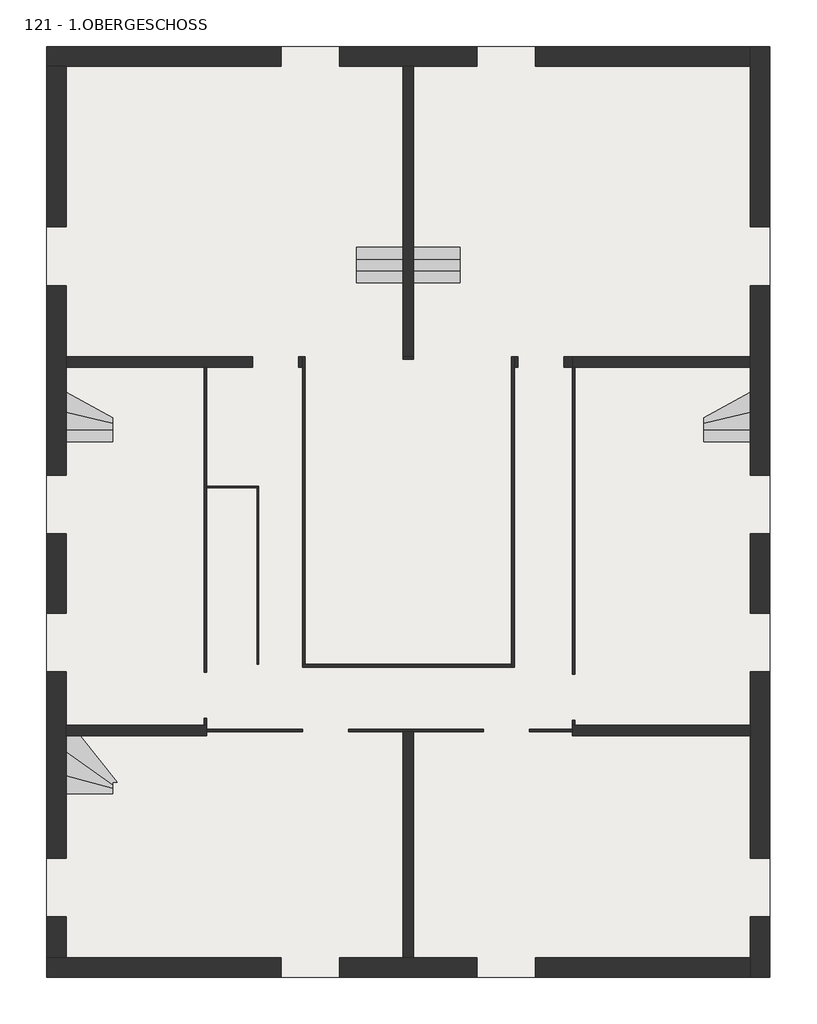
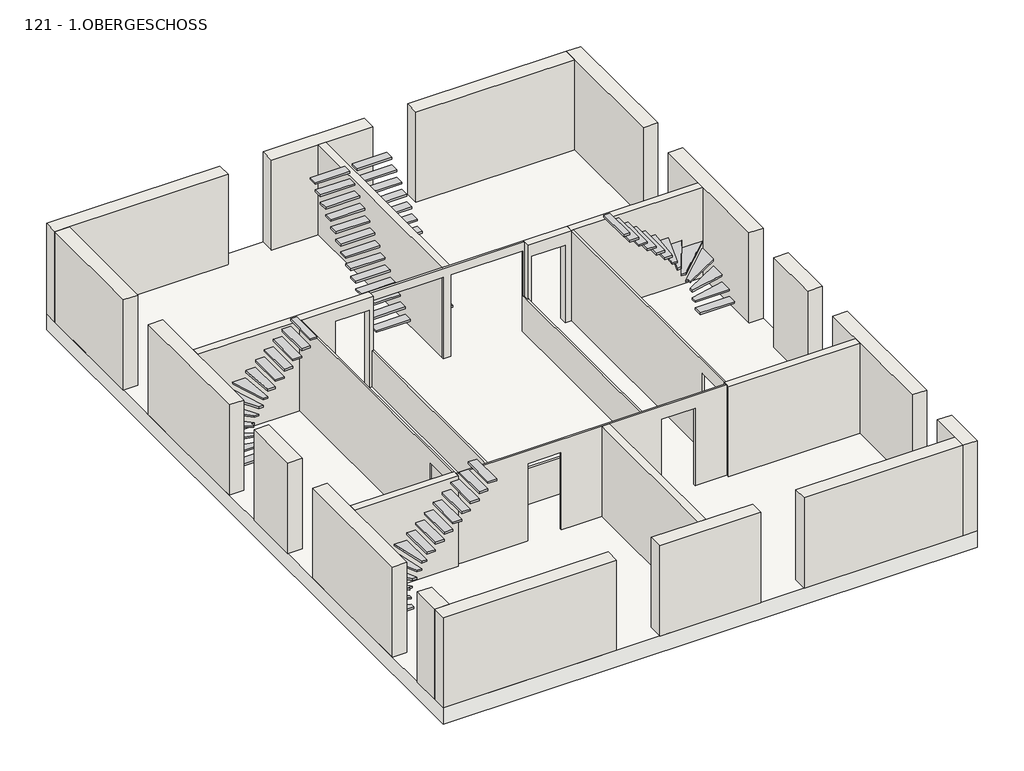
# One storey: 20 walls, 10 stairs, 1 slab.
# Revit data of these elements (continued)
# Type "  97010 :   97010" (continued)
#   Allright_Bauteil_ID = "0121Tre0785086959"
#   Material = "Stahlbeton"
#   Objektname = "Treppe"
#   NameOverride = " "
#   ThermalTransmittance = 0.0000 BTU/(h·ft²·°F)
#   NosingLength = 0.000 m
#   NumberOfRiser = 14
#   NumberOfTreads = 14
#   RiserHeight = 2.000 m
#   TreadLength = 2.300 m
#   IsExternal = no
#   FireExit = no
#   HandicapAccessible = no
#   HasNonSkidSurface = no
# Type "  97882 :   97882"
#   Abrechnungsart = "St"
#   Allright_Bauteil_ID = "0121Tre0785065280"
#   Codetext = "TR-MASSIV-GER\\"
#   Material = "Stahlbeton"
#   Objektname = "Treppe"
#   NameOverride = " "
#   Reference = "STB-Treppe"
#   ThermalTransmittance = 0.0000 BTU/(h·ft²·°F)
#   NosingLength = 0.000 m
#   NumberOfRiser = 14
#   NumberOfTreads = 13
#   RiserHeight = 2.021 m
#   TreadLength = 2.300 m
#   IsExternal = no
#   FireExit = no
#   HandicapAccessible = no
#   HasNonSkidSurface = no
# Type "  98300 :   98300"
#   Abrechnungsart = "St"
#   Allright_Bauteil_ID = "0121Tre0785065278"
#   Codetext = "TR-MASSIV-GER\\"
#   Material = "Stahlbeton"
#   Objektname = "Treppe"
#   NameOverride = " "
#   Reference = "STB-Treppe"
#   ThermalTransmittance = 0.0000 BTU/(h·ft²·°F)
#   NosingLength = 0.000 m
#   NumberOfRiser = 14
#   NumberOfTreads = 13
#   RiserHeight = 2.021 m
#   TreadLength = 2.300 m
#   IsExternal = no
#   FireExit = no
#   HandicapAccessible = no
#   HasNonSkidSurface = no
# Type "  98728 :   98728"
#   Abrechnungsart = "St"
#   Allright_Bauteil_ID = "0121Tre0785070507"
#   Material = "Stahlbeton"
#   Objektname = "Treppe"
#   NameOverride = " "
#   ThermalTransmittance = 0.0000 BTU/(h·ft²·°F)
#   NosingLength = 0.000 m
#   NumberOfRiser = 14
#   NumberOfTreads = 13
#   RiserHeight = 2.021 m
#   TreadLength = 2.300 m
#   IsExternal = no
#   FireExit = no
#   HandicapAccessible = no
#   HasNonSkidSurface = no
# Type "  99154 :   99154"
#   Abrechnungsart = "St"
#   Allright_Bauteil_ID = "0121Tre0785070829"
#   Material = "Stahlbeton"
#   Objektname = "Treppe"
#   NameOverride = " "
#   ThermalTransmittance = 0.0000 BTU/(h·ft²·°F)
#   NosingLength = 0.000 m
#   NumberOfRiser = 14
#   NumberOfTreads = 13
#   RiserHeight = 2.021 m
#   TreadLength = 2.300 m
#   IsExternal = no
#   FireExit = no
#   HandicapAccessible = no
#   HasNonSkidSurface = no
# Type "  149542 :   149542"
#   Abrechnungsart = "St"
#   Allright_Bauteil_ID = "0131Tre0659044515"
#   Material = "Stahlbeton"
#   Objektname = "Treppe"
#   NameOverride = " "
#   ThermalTransmittance = 0.0000 BTU/(h·ft²·°F)
#   NosingLength = 0.000 m
#   NumberOfRiser = 14
#   NumberOfTreads = 14
#   RiserHeight = 2.000 m
#   TreadLength = 2.300 m
#   IsExternal = no
#   FireExit = no
#   HandicapAccessible = no
#   HasNonSkidSurface = no
# Type "  150414 :   150414"
#   Abrechnungsart = "St"
#   Allright_Bauteil_ID = "0131Tre0659044575"
#   Codetext = "TR-MASSIV-GER\\"
#   Material = "Stahlbeton"
#   Objektname = "Treppe"
#   NameOverride = " "
#   Reference = "STB-Treppe"
#   ThermalTransmittance = 0.0000 BTU/(h·ft²·°F)
#   NosingLength = 0.000 m
#   NumberOfRiser = 14
#   NumberOfTreads = 13
#   RiserHeight = 2.021 m
#   TreadLength = 2.300 m
#   IsExternal = no
#   FireExit = no
#   HandicapAccessible = no
#   HasNonSkidSurface = no
# Type "  150832 :   150832"
#   Abrechnungsart = "St"
#   Allright_Bauteil_ID = "0131Tre0659044593"
#   Codetext = "TR-MASSIV-GER\\"
#   Material = "Stahlbeton"
#   Objektname = "Treppe"
#   NameOverride = " "
#   Reference = "STB-Treppe"
#   ThermalTransmittance = 0.0000 BTU/(h·ft²·°F)
#   NosingLength = 0.000 m
#   NumberOfRiser = 14
#   NumberOfTreads = 13
#   RiserHeight = 2.021 m
#   TreadLength = 2.300 m
#   IsExternal = no
#   FireExit = no
#   HandicapAccessible = no
#   HasNonSkidSurface = no
# Type "  151260 :   151260"
#   Abrechnungsart = "St"
#   Allright_Bauteil_ID = "0131Tre0659044533"
#   Material = "Stahlbeton"
#   Objektname = "Treppe"
#   NameOverride = " "
#   ThermalTransmittance = 0.0000 BTU/(h·ft²·°F)
#   NosingLength = 0.000 m
#   NumberOfRiser = 14
#   NumberOfTreads = 13
#   RiserHeight = 2.021 m
#   TreadLength = 2.300 m
#   IsExternal = no
#   FireExit = no
#   HandicapAccessible = no
#   HasNonSkidSurface = no
# Type "  151686 :   151686"
#   Abrechnungsart = "St"
#   Allright_Bauteil_ID = "0131Tre0659044570"
#   Material = "Stahlbeton"
#   Objektname = "Treppe"
#   NameOverride = " "
#   ThermalTransmittance = 0.0000 BTU/(h·ft²·°F)
#   NosingLength = 0.000 m
#   NumberOfRiser = 14
#   NumberOfTreads = 13
#   RiserHeight = 2.021 m
#   TreadLength = 2.300 m
#   IsExternal = no
#   FireExit = no
#   HandicapAccessible = no
#   HasNonSkidSurface = no
# Type " :1166"
#   Layers, outside or top first: 0.050 m "glas" (function 1)
# Type "Holzwand:1150"
#   ThermalTransmittance = 0.0000 BTU/(h·ft²·°F)
#   Combustible = no
#   Compartmentation = no
#   Layers, outside or top first: 0.200 m "holzschalung" (function 1)
# Type "Holzwand:1151"
#   ThermalTransmittance = 0.0000 BTU/(h·ft²·°F)
#   Combustible = no
#   Compartmentation = no
#   Layers, outside or top first: 0.200 m "holzschalung" (function 1)
# Type "Holzwand:1153"
#   ThermalTransmittance = 0.0000 BTU/(h·ft²·°F)
#   Combustible = no
#   Compartmentation = no
#   Layers, outside or top first: 0.200 m "holzschalung" (function 1)
# Type "Holzwand:1154"
#   ThermalTransmittance = 0.0000 BTU/(h·ft²·°F)
#   Combustible = no
#   Compartmentation = no
#   Layers, outside or top first: 0.030 m "holzschalung" (function 1)
# Type "Holzwand:1155"
#   ThermalTransmittance = 0.0000 BTU/(h·ft²·°F)
#   Combustible = no
#   Compartmentation = no
#   Layers, outside or top first: 0.030 m "holzschalung" (function 1)
# Type "1186 Atriumwand"
#   Layers, outside or top first: 0.050 m "holzschalung" (function 1)
# Type "Holzwand:1157"
#   ThermalTransmittance = 0.0000 BTU/(h·ft²·°F)
#   Combustible = no
#   Compartmentation = no
#   Layers, outside or top first: 0.200 m "holzschalung" (function 1)
# Type "Holzwand:1160"
#   ThermalTransmittance = 0.0000 BTU/(h·ft²·°F)
#   Combustible = no
#   Compartmentation = no
#   Layers, outside or top first: 0.200 m "holzschalung" (function 1)
# Type "Holzwand:1162"
#   ThermalTransmittance = 0.0000 BTU/(h·ft²·°F)
#   Combustible = no
#   Compartmentation = no
#   Layers, outside or top first: 0.200 m "holzschalung" (function 1)
# Type "Holzwand:1163"
#   ThermalTransmittance = 0.0000 BTU/(h·ft²·°F)
#   Combustible = no
#   Compartmentation = no
#   Layers, outside or top first: 0.200 m "holzschalung" (function 1)
# Type " :1167"
#   Layers, outside or top first: 0.050 m "holzschalung" (function 1)
# Type " :1168"
#   Layers, outside or top first: 0.050 m "holzschalung" (function 1)
# Type " :1169"
#   Layers, outside or top first: 0.050 m "holzschalung" (function 1)
# Type "1141 Aussenwand"
#   Layers, outside or top first: 0.380 m "holzschalung" (function 1)
# Element 1 (IfcSlab, "Holzdecke 176 : Holzdecke 176")
#   IFC Predefined Type = "FLOOR"
#   Export to IFC As = "ifcslab"
#   IfcGUID = "1_9Us2eVX4OuIZjhNyqdxW"
#   Phase Created = New Construction
#   Materials on its faces: "holzschalung"
# Element 2 (IfcStair, "  97010 :   97010")
#   IFC Predefined Type = "NOTDEFINED"
#   Export to IFC As = "ifcstair"
#   IfcGUID = "2ccaodaeb6QgHPV1d4NBnA"
#   Phase Created = New Construction
#   Materials on its faces: "weiss"
# Element 3 (IfcStair, "  97882 :   97882")
#   IFC Predefined Type = "STRAIGHT_RUN_STAIR"
#   Export to IFC As = "ifcstair"
#   IfcGUID = "1nghyUHoH9yBc_lxkBTUjw"
#   Phase Created = New Construction
#   Materials on its faces: "weiss"
# Element 4 (IfcStair, "  98300 :   98300")
#   IFC Predefined Type = "STRAIGHT_RUN_STAIR"
#   Export to IFC As = "ifcstair"
#   IfcGUID = "2AC_Gmfhz1LvYwUyPOxWan"
#   Phase Created = New Construction
#   Materials on its faces: "weiss"
# Element 5 (IfcStair, "  98728 :   98728")
#   IFC Predefined Type = "NOTDEFINED"
#   Export to IFC As = "ifcstair"
#   IfcGUID = "04Edcgbk9CPwWYiYhycXFf"
#   Phase Created = New Construction
#   Materials on its faces: "weiss"
# Element 6 (IfcStair, "  99154 :   99154")
#   IFC Predefined Type = "NOTDEFINED"
#   Export to IFC As = "ifcstair"
#   IfcGUID = "1azVXxNdn2POY9VYN93ccY"
#   Phase Created = New Construction
#   Materials on its faces: "weiss"
# Element 7 (IfcStair, "  149542 :   149542")
#   IFC Predefined Type = "NOTDEFINED"
#   Export to IFC As = "ifcstair"
#   IfcGUID = "1sH4rJKnLAFOtHPnXrLkif"
#   Phase Created = New Construction
#   Materials on its faces: "weiss"
# Element 8 (IfcStair, "  150414 :   150414")
#   IFC Predefined Type = "STRAIGHT_RUN_STAIR"
#   Export to IFC As = "ifcstair"
#   IfcGUID = "3fdccs_Mj1YAyFFpBc3gyk"
#   Phase Created = New Construction
#   Materials on its faces: "weiss"
# Element 9 (IfcStair, "  150832 :   150832")
#   IFC Predefined Type = "STRAIGHT_RUN_STAIR"
#   Export to IFC As = "ifcstair"
#   IfcGUID = "2szmEZdbD3KBDvfX1Sa6Vh"
#   Phase Created = New Construction
#   Materials on its faces: "weiss"
# Element 10 (IfcStair, "  151260 :   151260")
#   IFC Predefined Type = "NOTDEFINED"
#   Export to IFC As = "ifcstair"
#   IfcGUID = "1YKyaFTbr8YR41yGjubBsl"
#   Phase Created = New Construction
#   Materials on its faces: "weiss"
# Element 11 (IfcStair, "  151686 :   151686")
#   IFC Predefined Type = "NOTDEFINED"
#   Export to IFC As = "ifcstair"
#   IfcGUID = "2KPGRYHzzCygzBebAeLtPz"
#   Phase Created = New Construction
#   Materials on its faces: "weiss"
# Element 12 (IfcWall, " :1166")
#   Export to IFC As = "ifcwall"
#   IfcGUID = "0t2qqx1kvDZPNPdKl4bfzP"
#   NameOverride = " "
#   Abrechnungsart = "m³"
#   Allright_Bauteil_ID = "0121HWa0785064296"
#   Layer #1:Object Layer Attributes #1:Abrechnungsart = "m²"
#   Layer #1:Object Layer Attributes #1:Allright_Bauteil_ID = "0121Wa 0785064386"
#   Layer #1:Object Layer Attributes #1:Gewerk = "Zimmer- und Holzbauarbeiten"
#   Layer #1:Object Layer Attributes #1:Material = "k.Ausw."
#   Layer #1:Object Layer Attributes #1:Objektname = "Wand"
#   Layer #1:Object Layer Attributes #1:Status = "Neubau"
#   MEP Wandtyp = "HO-WA-HSW\\"
#   Objektname = "Gesamtwand"
#   built-in parameter 1001111 = 0.505 m
#   Top Offset = 0.000 m
#   Base Offset = 0.505 m
#   Unconnected Height = 2.500 m
#   wall height = 2.500 m
#   Layer #1:Object Layer Attributes #1:2D Interaktion = yes
#   Phase Created = New Construction
#   Base Constraint = 121 - 1.OBERGESCHOSS
#   Materials on its faces: "glas"
# Element 13 (IfcWall, "Holzwand:1150")
#   Export to IFC As = "ifcwall"
#   IfcGUID = "3nZ5Mon9nBjwoRgvyoor9a"
#   NameOverride = "Holzwand"
#   Abrechnungsart = "St"
#   Allright_Bauteil_ID = "0121HWa0785065367"
#   Bezeichnung = "Holzwand"
#   Layer #1:Object Layer Attributes #1:Abrechnungsart = "m²"
#   Layer #1:Object Layer Attributes #1:Allright_Bauteil_ID = "0121Wa 0785065369"
#   Layer #1:Object Layer Attributes #1:Bezeichnung = "Holzwand"
#   Layer #1:Object Layer Attributes #1:Codetext = "HO-WI-HSW\\"
#   Layer #1:Object Layer Attributes #1:Gewerk = "Zimmer- und Holzbauarbeiten"
#   Layer #1:Object Layer Attributes #1:Material = "Holz"
#   Layer #1:Object Layer Attributes #1:Objektname = "Wand"
#   Layer #1:Object Layer Attributes #1:Reference = "Holzwand"
#   Layer #1:Object Layer Attributes #1:Status = "Neubau"
#   MEP Wandtyp = "HO-WA-HSW\\"
#   Objektname = "Gesamtwand"
#   Reference = "Holzwand"
#   Status = "NEW"
#   built-in parameter 1001111 = 0.505 m
#   Top Offset = 0.000 m
#   Base Offset = 0.505 m
#   Unconnected Height = 2.500 m
#   wall height = 2.500 m
#   Layer #1:Object Layer Attributes #1:U-Wert = 0
#   Layer #1:Object Layer Attributes #1:2D Interaktion = yes
#   Layer #1:Object Layer Attributes #1:Außenbauteil = no
#   Layer #1:Object Layer Attributes #1:Brandabschnittsdefinierendes Bauteil = no
#   Layer #1:Object Layer Attributes #1:Brennbares Material = no
#   Layer #1:Object Layer Attributes #1:Raumhohe Wand = yes
#   Layer #1:Object Layer Attributes #1:Tragendes Bauteil = yes
#   ExtendToStructure = yes
#   IsExternal = no
#   LoadBearing = yes
#   Phase Created = New Construction
#   Base Constraint = 121 - 1.OBERGESCHOSS
#   Materials on its faces: "holzschalung"
# Element 14 (IfcWall, "Holzwand:1151")
#   Export to IFC As = "ifcwall"
#   IfcGUID = "3jE1E$NFj7vAP$vn70kdrt"
#   NameOverride = "Holzwand"
#   Abrechnungsart = "St"
#   Allright_Bauteil_ID = "0121HWa0785066899"
#   Bezeichnung = "Holzwand"
#   Layer #1:Object Layer Attributes #1:Abrechnungsart = "m²"
#   Layer #1:Object Layer Attributes #1:Allright_Bauteil_ID = "0121Wa 0785066901"
#   Layer #1:Object Layer Attributes #1:Bezeichnung = "Holzwand"
#   Layer #1:Object Layer Attributes #1:Codetext = "HO-WI-HSW\\"
#   Layer #1:Object Layer Attributes #1:Gewerk = "Zimmer- und Holzbauarbeiten"
#   Layer #1:Object Layer Attributes #1:Material = "Holz"
#   Layer #1:Object Layer Attributes #1:Objektname = "Wand"
#   Layer #1:Object Layer Attributes #1:Reference = "Holzwand"
#   Layer #1:Object Layer Attributes #1:Status = "Neubau"
#   MEP Wandtyp = "HO-WA-HSW\\"
#   Objektname = "Gesamtwand"
#   Reference = "Holzwand"
#   Status = "NEW"
#   built-in parameter 1001111 = 0.505 m
#   Top Offset = 0.000 m
#   Base Offset = 0.505 m
#   Unconnected Height = 2.500 m
#   wall height = 2.500 m
#   Layer #1:Object Layer Attributes #1:U-Wert = 0
#   Layer #1:Object Layer Attributes #1:2D Interaktion = yes
#   Layer #1:Object Layer Attributes #1:Außenbauteil = no
#   Layer #1:Object Layer Attributes #1:Brandabschnittsdefinierendes Bauteil = no
#   Layer #1:Object Layer Attributes #1:Brennbares Material = no
#   Layer #1:Object Layer Attributes #1:Raumhohe Wand = yes
#   Layer #1:Object Layer Attributes #1:Tragendes Bauteil = yes
#   ExtendToStructure = yes
#   IsExternal = no
#   LoadBearing = yes
#   Phase Created = New Construction
#   Base Constraint = 121 - 1.OBERGESCHOSS
#   Materials on its faces: "holzschalung"
# Element 15 (IfcWall, "Holzwand:1153")
#   Export to IFC As = "ifcwall"
#   IfcGUID = "1Zhxv5EALB9e6_$pCtUEXg"
#   NameOverride = "Holzwand"
#   Abrechnungsart = "St"
#   Allright_Bauteil_ID = "0121HWa0785065540"
#   Bezeichnung = "Holzwand"
#   Layer #1:Object Layer Attributes #1:Abrechnungsart = "m²"
#   Layer #1:Object Layer Attributes #1:Allright_Bauteil_ID = "0121Wa 0785065541"
#   Layer #1:Object Layer Attributes #1:Bezeichnung = "Holzwand"
#   Layer #1:Object Layer Attributes #1:Codetext = "HO-WI-HSW\\"
#   Layer #1:Object Layer Attributes #1:Gewerk = "Zimmer- und Holzbauarbeiten"
#   Layer #1:Object Layer Attributes #1:Material = "Holz"
#   Layer #1:Object Layer Attributes #1:Objektname = "Wand"
#   Layer #1:Object Layer Attributes #1:Reference = "Holzwand"
#   Layer #1:Object Layer Attributes #1:Status = "Neubau"
#   MEP Wandtyp = "HO-WA-HSW\\"
#   Objektname = "Gesamtwand"
#   Reference = "Holzwand"
#   Status = "NEW"
#   built-in parameter 1001111 = 0.505 m
#   Top Offset = 0.000 m
#   Base Offset = 0.505 m
#   Unconnected Height = 2.500 m
#   wall height = 2.500 m
#   Layer #1:Object Layer Attributes #1:U-Wert = 0
#   Layer #1:Object Layer Attributes #1:2D Interaktion = yes
#   Layer #1:Object Layer Attributes #1:Außenbauteil = no
#   Layer #1:Object Layer Attributes #1:Brandabschnittsdefinierendes Bauteil = no
#   Layer #1:Object Layer Attributes #1:Brennbares Material = no
#   Layer #1:Object Layer Attributes #1:Raumhohe Wand = yes
#   Layer #1:Object Layer Attributes #1:Tragendes Bauteil = yes
#   ExtendToStructure = yes
#   IsExternal = no
#   LoadBearing = yes
#   Phase Created = New Construction
#   Base Constraint = 121 - 1.OBERGESCHOSS
#   Materials on its faces: "holzschalung"
# Element 16 (IfcWall, "Holzwand:1154")
#   Export to IFC As = "ifcwall"
#   IfcGUID = "2MsVq3EJn0K8wHdQ6uoxnd"
#   NameOverride = "Holzwand"
#   Abrechnungsart = "St"
#   Allright_Bauteil_ID = "0121HWa0785067355"
#   Bezeichnung = "Holzwand"
#   Layer #1:Object Layer Attributes #1:Abrechnungsart = "m²"
#   Layer #1:Object Layer Attributes #1:Allright_Bauteil_ID = "0121Wa 0785067356"
#   Layer #1:Object Layer Attributes #1:Codetext = "HO-WI-HSW\\"
#   Layer #1:Object Layer Attributes #1:Gewerk = "Zimmer- und Holzbauarbeiten"
#   Layer #1:Object Layer Attributes #1:Material = "Holz"
#   Layer #1:Object Layer Attributes #1:Objektname = "Wand"
#   Layer #1:Object Layer Attributes #1:Reference = "Holzwand"
#   Layer #1:Object Layer Attributes #1:Status = "Neubau"
#   MEP Wandtyp = "HO-WA-HSW\\"
#   Objektname = "Gesamtwand"
#   Reference = "Holzwand"
#   Status = "NEW"
#   built-in parameter 1001111 = 0.505 m
#   Top Offset = 0.000 m
#   Base Offset = 0.505 m
#   Unconnected Height = 1.000 m
#   wall height = 1.000 m
#   Layer #1:Object Layer Attributes #1:U-Wert = 0
#   Layer #1:Object Layer Attributes #1:2D Interaktion = yes
#   Layer #1:Object Layer Attributes #1:Außenbauteil = no
#   Layer #1:Object Layer Attributes #1:Brandabschnittsdefinierendes Bauteil = no
#   Layer #1:Object Layer Attributes #1:Brennbares Material = no
#   Layer #1:Object Layer Attributes #1:Raumhohe Wand = yes
#   ExtendToStructure = yes
#   IsExternal = no
#   LoadBearing = yes
#   Phase Created = New Construction
#   Base Constraint = 121 - 1.OBERGESCHOSS
#   Materials on its faces: "holzschalung"
# Element 17 (IfcWall, "Holzwand:1155")
#   Export to IFC As = "ifcwall"
#   IfcGUID = "1F_ySrDsP9oP3MqXymSTVO"
#   NameOverride = "Holzwand"
#   Abrechnungsart = "St"
#   Allright_Bauteil_ID = "0121HWa0785067347"
#   Bezeichnung = "Holzwand"
#   Layer #1:Object Layer Attributes #1:Abrechnungsart = "m²"
#   Layer #1:Object Layer Attributes #1:Allright_Bauteil_ID = "0121Wa 0785067348"
#   Layer #1:Object Layer Attributes #1:Codetext = "HO-WI-HSW\\"
#   Layer #1:Object Layer Attributes #1:Gewerk = "Zimmer- und Holzbauarbeiten"
#   Layer #1:Object Layer Attributes #1:Material = "Holz"
#   Layer #1:Object Layer Attributes #1:Objektname = "Wand"
#   Layer #1:Object Layer Attributes #1:Reference = "Holzwand"
#   Layer #1:Object Layer Attributes #1:Status = "Neubau"
#   MEP Wandtyp = "HO-WA-HSW\\"
#   Objektname = "Gesamtwand"
#   Reference = "Holzwand"
#   Status = "NEW"
#   built-in parameter 1001111 = 0.505 m
#   Top Offset = 0.000 m
#   Base Offset = 0.505 m
#   Unconnected Height = 1.000 m
#   wall height = 1.000 m
#   Layer #1:Object Layer Attributes #1:U-Wert = 0
#   Layer #1:Object Layer Attributes #1:2D Interaktion = yes
#   Layer #1:Object Layer Attributes #1:Außenbauteil = no
#   Layer #1:Object Layer Attributes #1:Brandabschnittsdefinierendes Bauteil = no
#   Layer #1:Object Layer Attributes #1:Brennbares Material = no
#   Layer #1:Object Layer Attributes #1:Raumhohe Wand = yes
#   ExtendToStructure = yes
#   IsExternal = no
#   LoadBearing = yes
#   Phase Created = New Construction
#   Base Constraint = 121 - 1.OBERGESCHOSS
#   Materials on its faces: "holzschalung"
# Element 18 (IfcWall, "1186 Atriumwand")
#   Export to IFC As = "ifcwall"
#   IfcGUID = "0gtwZwppj1pObqyI7HY41_"
#   NameOverride = "Holzwand"
#   Abrechnungsart = "St"
#   Allright_Bauteil_ID = "0121HWa0785064323"
#   Bezeichnung = "Holzwand"
#   Layer #1:Object Layer Attributes #1:Abrechnungsart = "m²"
#   Layer #1:Object Layer Attributes #1:Allright_Bauteil_ID = "0121Wa 0785064369"
#   Layer #1:Object Layer Attributes #1:Bezeichnung = "Holzwand"
#   Layer #1:Object Layer Attributes #1:Codetext = "HO-WI-HSW\\"
#   Layer #1:Object Layer Attributes #1:Gewerk = "Zimmer- und Holzbauarbeiten"
#   Layer #1:Object Layer Attributes #1:Material = "Holz"
#   Layer #1:Object Layer Attributes #1:Objektname = "Wand"
#   Layer #1:Object Layer Attributes #1:Reference = "Holzwand"
#   Layer #1:Object Layer Attributes #1:Status = "Neubau"
#   MEP Wandtyp = "HO-WA-HSW\\"
#   Objektname = "Gesamtwand"
#   Reference = "Holzwand"
#   Status = "NEW"
#   built-in parameter 1001111 = 0.505 m
#   Top Offset = 0.000 m
#   Base Offset = 0.505 m
#   Unconnected Height = 2.500 m
#   wall height = 2.500 m
#   Layer #1:Object Layer Attributes #1:U-Wert = 0
#   Layer #1:Object Layer Attributes #1:2D Interaktion = yes
#   Layer #1:Object Layer Attributes #1:Außenbauteil = no
#   Layer #1:Object Layer Attributes #1:Brandabschnittsdefinierendes Bauteil = no
#   Layer #1:Object Layer Attributes #1:Brennbares Material = no
#   Layer #1:Object Layer Attributes #1:Raumhohe Wand = yes
#   Layer #1:Object Layer Attributes #1:Tragendes Bauteil = yes
#   ExtendToStructure = yes
#   IsExternal = no
#   LoadBearing = yes
#   Phase Created = New Construction
#   Base Constraint = 121 - 1.OBERGESCHOSS
#   Materials on its faces: "holzschalung"
# Element 19 (IfcWall, "Holzwand:1157")
#   Export to IFC As = "ifcwall"
#   IfcGUID = "0tY6$O1l121AktLhYSWZjf"
#   NameOverride = "Holzwand"
#   Abrechnungsart = "St"
#   Allright_Bauteil_ID = "0121HWa0785064381"
#   Bezeichnung = "Holzwand"
#   Layer #1:Object Layer Attributes #1:Abrechnungsart = "m²"
#   Layer #1:Object Layer Attributes #1:Allright_Bauteil_ID = "0121Wa 0785064384"
#   Layer #1:Object Layer Attributes #1:Bezeichnung = "Holzwand"
#   Layer #1:Object Layer Attributes #1:Codetext = "HO-WI-HSW\\"
#   Layer #1:Object Layer Attributes #1:Gewerk = "Zimmer- und Holzbauarbeiten"
#   Layer #1:Object Layer Attributes #1:Material = "Holz"
#   Layer #1:Object Layer Attributes #1:Objektname = "Wand"
#   Layer #1:Object Layer Attributes #1:Reference = "Holzwand"
#   Layer #1:Object Layer Attributes #1:Status = "Neubau"
#   MEP Wandtyp = "HO-WA-HSW\\"
#   Objektname = "Gesamtwand"
#   Reference = "Holzwand"
#   Status = "NEW"
#   built-in parameter 1001111 = 0.505 m
#   Top Offset = 0.000 m
#   Base Offset = 0.505 m
#   Unconnected Height = 2.500 m
#   wall height = 2.500 m
#   Layer #1:Object Layer Attributes #1:U-Wert = 0
#   Layer #1:Object Layer Attributes #1:2D Interaktion = yes
#   Layer #1:Object Layer Attributes #1:Außenbauteil = no
#   Layer #1:Object Layer Attributes #1:Brandabschnittsdefinierendes Bauteil = no
#   Layer #1:Object Layer Attributes #1:Brennbares Material = no
#   Layer #1:Object Layer Attributes #1:Raumhohe Wand = yes
#   Layer #1:Object Layer Attributes #1:Tragendes Bauteil = yes
#   ExtendToStructure = yes
#   IsExternal = no
#   LoadBearing = yes
#   Phase Created = New Construction
#   Base Constraint = 121 - 1.OBERGESCHOSS
#   Materials on its faces: "holzschalung"
# Element 20 (IfcWall, "1186 Atriumwand")
#   Export to IFC As = "ifcwall"
#   IfcGUID = "2Mr8L52dj4iP8MoJTiOa9p"
#   NameOverride = "Holzwand"
#   Abrechnungsart = "St"
#   Allright_Bauteil_ID = "0121HWa0785069286"
#   Bezeichnung = "Holzwand"
#   Layer #1:Object Layer Attributes #1:Abrechnungsart = "m²"
#   Layer #1:Object Layer Attributes #1:Allright_Bauteil_ID = "0121Wa 0785069294"
#   Layer #1:Object Layer Attributes #1:Bezeichnung = "Holzwand"
#   Layer #1:Object Layer Attributes #1:Codetext = "HO-WI-HSW\\"
#   Layer #1:Object Layer Attributes #1:Gewerk = "Zimmer- und Holzbauarbeiten"
#   Layer #1:Object Layer Attributes #1:Material = "Holz"
#   Layer #1:Object Layer Attributes #1:Objektname = "Wand"
#   Layer #1:Object Layer Attributes #1:Reference = "Holzwand"
#   Layer #1:Object Layer Attributes #1:Status = "Neubau"
#   MEP Wandtyp = "HO-WA-HSW\\"
#   Objektname = "Gesamtwand"
#   Reference = "Holzwand"
#   Status = "NEW"
#   built-in parameter 1001111 = 0.505 m
#   Top Offset = 0.000 m
#   Base Offset = 0.505 m
#   Unconnected Height = 2.500 m
#   wall height = 2.500 m
#   Layer #1:Object Layer Attributes #1:U-Wert = 0
#   Layer #1:Object Layer Attributes #1:2D Interaktion = yes
#   Layer #1:Object Layer Attributes #1:Außenbauteil = no
#   Layer #1:Object Layer Attributes #1:Brandabschnittsdefinierendes Bauteil = no
#   Layer #1:Object Layer Attributes #1:Brennbares Material = no
#   Layer #1:Object Layer Attributes #1:Raumhohe Wand = yes
#   Layer #1:Object Layer Attributes #1:Tragendes Bauteil = yes
#   ExtendToStructure = yes
#   IsExternal = no
#   LoadBearing = yes
#   Phase Created = New Construction
#   Base Constraint = 121 - 1.OBERGESCHOSS
#   Materials on its faces: "holzschalung"
# Element 21 (IfcWall, "1186 Atriumwand")
#   Export to IFC As = "ifcwall"
#   IfcGUID = "36leNf4gL9OB_v358ffY76"
#   NameOverride = "Holzwand"
#   Abrechnungsart = "St"
#   Allright_Bauteil_ID = "0121HWa0785064324"
#   Bezeichnung = "Holzwand"
#   Layer #1:Object Layer Attributes #1:Abrechnungsart = "m²"
#   Layer #1:Object Layer Attributes #1:Allright_Bauteil_ID = "0121Wa 0785064395"
#   Layer #1:Object Layer Attributes #1:Bezeichnung = "Holzwand"
#   Layer #1:Object Layer Attributes #1:Codetext = "HO-WI-HSW\\"
#   Layer #1:Object Layer Attributes #1:Gewerk = "Zimmer- und Holzbauarbeiten"
#   Layer #1:Object Layer Attributes #1:Material = "Holz"
#   Layer #1:Object Layer Attributes #1:Objektname = "Wand"
#   Layer #1:Object Layer Attributes #1:Reference = "Holzwand"
#   Layer #1:Object Layer Attributes #1:Status = "Neubau"
#   MEP Wandtyp = "HO-WA-HSW\\"
#   Objektname = "Gesamtwand"
#   Reference = "Holzwand"
#   Status = "NEW"
#   built-in parameter 1001111 = 0.505 m
#   Top Offset = 0.000 m
#   Base Offset = 0.505 m
#   Unconnected Height = 2.500 m
#   wall height = 2.500 m
#   Layer #1:Object Layer Attributes #1:U-Wert = 0
#   Layer #1:Object Layer Attributes #1:2D Interaktion = yes
#   Layer #1:Object Layer Attributes #1:Außenbauteil = no
#   Layer #1:Object Layer Attributes #1:Brandabschnittsdefinierendes Bauteil = no
#   Layer #1:Object Layer Attributes #1:Brennbares Material = no
#   Layer #1:Object Layer Attributes #1:Raumhohe Wand = yes
#   Layer #1:Object Layer Attributes #1:Tragendes Bauteil = yes
#   ExtendToStructure = yes
#   IsExternal = no
#   LoadBearing = yes
#   Phase Created = New Construction
#   Base Constraint = 121 - 1.OBERGESCHOSS
#   Materials on its faces: "holzschalung"
# Element 22 (IfcWall, "Holzwand:1160")
#   Export to IFC As = "ifcwall"
#   IfcGUID = "3kHHpx_NTE_9JnfL3dFkYB"
#   NameOverride = "Holzwand"
#   Abrechnungsart = "St"
#   Allright_Bauteil_ID = "0121HWa0785064389"
#   Bezeichnung = "Holzwand"
#   Layer #1:Object Layer Attributes #1:Abrechnungsart = "m²"
#   Layer #1:Object Layer Attributes #1:Allright_Bauteil_ID = "0121Wa 0785064393"
#   Layer #1:Object Layer Attributes #1:Bezeichnung = "Holzwand"
#   Layer #1:Object Layer Attributes #1:Codetext = "HO-WI-HSW\\"
#   Layer #1:Object Layer Attributes #1:Gewerk = "Zimmer- und Holzbauarbeiten"
#   Layer #1:Object Layer Attributes #1:Material = "Holz"
#   Layer #1:Object Layer Attributes #1:Objektname = "Wand"
#   Layer #1:Object Layer Attributes #1:Reference = "Holzwand"
#   Layer #1:Object Layer Attributes #1:Status = "Neubau"
#   MEP Wandtyp = "HO-WA-HSW\\"
#   Objektname = "Gesamtwand"
#   Reference = "Holzwand"
#   Status = "NEW"
#   built-in parameter 1001111 = 0.505 m
#   Top Offset = 0.000 m
#   Base Offset = 0.505 m
#   Unconnected Height = 2.500 m
#   wall height = 2.500 m
#   Layer #1:Object Layer Attributes #1:U-Wert = 0
#   Layer #1:Object Layer Attributes #1:2D Interaktion = yes
#   Layer #1:Object Layer Attributes #1:Außenbauteil = no
#   Layer #1:Object Layer Attributes #1:Brandabschnittsdefinierendes Bauteil = no
#   Layer #1:Object Layer Attributes #1:Brennbares Material = no
#   Layer #1:Object Layer Attributes #1:Raumhohe Wand = yes
#   Layer #1:Object Layer Attributes #1:Tragendes Bauteil = yes
#   ExtendToStructure = yes
#   IsExternal = no
#   LoadBearing = yes
#   Phase Created = New Construction
#   Base Constraint = 121 - 1.OBERGESCHOSS
#   Materials on its faces: "holzschalung"
# Element 23 (IfcWall, "Holzwand:1162")
#   Export to IFC As = "ifcwall"
#   IfcGUID = "26lQuimMP00PZvPhbBRI2R"
#   NameOverride = "Holzwand"
#   Abrechnungsart = "St"
#   Allright_Bauteil_ID = "0121HWa0785065329"
#   Bezeichnung = "Holzwand"
#   Layer #1:Object Layer Attributes #1:Abrechnungsart = "m²"
#   Layer #1:Object Layer Attributes #1:Allright_Bauteil_ID = "0121Wa 0785065331"
#   Layer #1:Object Layer Attributes #1:Bezeichnung = "Holzwand"
#   Layer #1:Object Layer Attributes #1:Codetext = "HO-WI-HSW\\"
#   Layer #1:Object Layer Attributes #1:Gewerk = "Zimmer- und Holzbauarbeiten"
#   Layer #1:Object Layer Attributes #1:Material = "Holz"
#   Layer #1:Object Layer Attributes #1:Objektname = "Wand"
#   Layer #1:Object Layer Attributes #1:Reference = "Holzwand"
#   Layer #1:Object Layer Attributes #1:Status = "Neubau"
#   MEP Wandtyp = "HO-WA-HSW\\"
#   Objektname = "Gesamtwand"
#   Reference = "Holzwand"
#   Status = "NEW"
#   built-in parameter 1001111 = 0.505 m
#   Top Offset = 0.000 m
#   Base Offset = 0.505 m
#   Unconnected Height = 2.500 m
#   wall height = 2.500 m
#   Layer #1:Object Layer Attributes #1:U-Wert = 0
#   Layer #1:Object Layer Attributes #1:2D Interaktion = yes
#   Layer #1:Object Layer Attributes #1:Außenbauteil = no
#   Layer #1:Object Layer Attributes #1:Brandabschnittsdefinierendes Bauteil = no
#   Layer #1:Object Layer Attributes #1:Brennbares Material = no
#   Layer #1:Object Layer Attributes #1:Raumhohe Wand = yes
#   Layer #1:Object Layer Attributes #1:Tragendes Bauteil = yes
#   ExtendToStructure = yes
#   IsExternal = no
#   LoadBearing = yes
#   Phase Created = New Construction
#   Base Constraint = 121 - 1.OBERGESCHOSS
#   Materials on its faces: "holzschalung"
# Element 24 (IfcWall, "Holzwand:1163")
#   Export to IFC As = "ifcwall"
#   IfcGUID = "3atU$IMTH8YP$GZozT8ehc"
#   NameOverride = "Holzwand"
#   Abrechnungsart = "St"
#   Allright_Bauteil_ID = "0121HWa0785064334"
#   Bezeichnung = "Holzwand"
#   Layer #1:Object Layer Attributes #1:Abrechnungsart = "m²"
#   Layer #1:Object Layer Attributes #1:Allright_Bauteil_ID = "0121Wa 0785064371"
#   Layer #1:Object Layer Attributes #1:Bezeichnung = "Holzwand"
#   Layer #1:Object Layer Attributes #1:Codetext = "HO-WI-HSW\\"
#   Layer #1:Object Layer Attributes #1:Gewerk = "Zimmer- und Holzbauarbeiten"
#   Layer #1:Object Layer Attributes #1:Material = "Holz"
#   Layer #1:Object Layer Attributes #1:Objektname = "Wand"
#   Layer #1:Object Layer Attributes #1:Reference = "Holzwand"
#   Layer #1:Object Layer Attributes #1:Status = "Neubau"
#   MEP Wandtyp = "HO-WA-HSW\\"
#   Objektname = "Gesamtwand"
#   Reference = "Holzwand"
#   Status = "NEW"
#   built-in parameter 1001111 = 0.505 m
#   Top Offset = 0.000 m
#   Base Offset = 0.505 m
#   Unconnected Height = 2.500 m
#   wall height = 2.500 m
#   Layer #1:Object Layer Attributes #1:U-Wert = 0
#   Layer #1:Object Layer Attributes #1:2D Interaktion = yes
#   Layer #1:Object Layer Attributes #1:Außenbauteil = no
#   Layer #1:Object Layer Attributes #1:Brandabschnittsdefinierendes Bauteil = no
#   Layer #1:Object Layer Attributes #1:Brennbares Material = no
#   Layer #1:Object Layer Attributes #1:Raumhohe Wand = yes
#   Layer #1:Object Layer Attributes #1:Tragendes Bauteil = yes
#   ExtendToStructure = yes
#   IsExternal = no
#   LoadBearing = yes
#   Phase Created = New Construction
#   Base Constraint = 121 - 1.OBERGESCHOSS
#   Materials on its faces: "holzschalung"
# Element 25 (IfcWall, " :1167")
#   Export to IFC As = "ifcwall"
#   IfcGUID = "35Iolt9MTFw82QPYPk5JvU"
#   NameOverride = " "
#   Abrechnungsart = "m³"
#   Allright_Bauteil_ID = "0121HWa0785064294"
#   Layer #1:Object Layer Attributes #1:Abrechnungsart = "m²"
#   Layer #1:Object Layer Attributes #1:Allright_Bauteil_ID = "0121Wa 0785064340"
#   Layer #1:Object Layer Attributes #1:Gewerk = "Zimmer- und Holzbauarbeiten"
#   Layer #1:Object Layer Attributes #1:Material = "k.Ausw."
#   Layer #1:Object Layer Attributes #1:Objektname = "Wand"
#   Layer #1:Object Layer Attributes #1:Status = "Neubau"
#   MEP Wandtyp = "HO-WA-HSW\\"
#   Objektname = "Gesamtwand"
#   built-in parameter 1001111 = 0.505 m
#   Top Offset = 0.000 m
#   Base Offset = 0.505 m
#   Unconnected Height = 1.000 m
#   wall height = 1.000 m
#   Layer #1:Object Layer Attributes #1:2D Interaktion = yes
#   Layer #1:Object Layer Attributes #1:Tragendes Bauteil = no
#   Phase Created = New Construction
#   Base Constraint = 121 - 1.OBERGESCHOSS
#   Materials on its faces: "holzschalung", "glas"
# Element 26 (IfcWall, " :1168")
#   Export to IFC As = "ifcwall"
#   IfcGUID = "21NDiotIv7sAO2c5Bbio25"
#   NameOverride = " "
#   Abrechnungsart = "m³"
#   Allright_Bauteil_ID = "0121HWa0785064290"
#   Layer #1:Object Layer Attributes #1:Abrechnungsart = "m²"
#   Layer #1:Object Layer Attributes #1:Allright_Bauteil_ID = "0121Wa 0785064348"
#   Layer #1:Object Layer Attributes #1:Gewerk = "Zimmer- und Holzbauarbeiten"
#   Layer #1:Object Layer Attributes #1:Material = "k.Ausw."
#   Layer #1:Object Layer Attributes #1:Objektname = "Wand"
#   Layer #1:Object Layer Attributes #1:Status = "Neubau"
#   MEP Wandtyp = "HO-WA-HSW\\"
#   Objektname = "Gesamtwand"
#   built-in parameter 1001111 = 0.505 m
#   Top Offset = 0.000 m
#   Base Offset = 0.505 m
#   Unconnected Height = 1.000 m
#   wall height = 1.000 m
#   Layer #1:Object Layer Attributes #1:2D Interaktion = yes
#   Layer #1:Object Layer Attributes #1:Tragendes Bauteil = no
#   Phase Created = New Construction
#   Base Constraint = 121 - 1.OBERGESCHOSS
#   Materials on its faces: "holzschalung"
# Element 27 (IfcWall, " :1169")
#   Export to IFC As = "ifcwall"
#   IfcGUID = "2aL_F8tebFMgUeEEKPH5KO"
#   NameOverride = " "
#   Abrechnungsart = "m³"
#   Allright_Bauteil_ID = "0121HWa0785064292"
#   Layer #1:Object Layer Attributes #1:Abrechnungsart = "m²"
#   Layer #1:Object Layer Attributes #1:Allright_Bauteil_ID = "0121Wa 0785064346"
#   Layer #1:Object Layer Attributes #1:Gewerk = "Zimmer- und Holzbauarbeiten"
#   Layer #1:Object Layer Attributes #1:Material = "k.Ausw."
#   Layer #1:Object Layer Attributes #1:Objektname = "Wand"
#   Layer #1:Object Layer Attributes #1:Status = "Neubau"
#   MEP Wandtyp = "HO-WA-HSW\\"
#   Objektname = "Gesamtwand"
#   built-in parameter 1001111 = 0.505 m
#   Top Offset = 0.000 m
#   Base Offset = 0.505 m
#   Unconnected Height = 1.000 m
#   wall height = 1.000 m
#   Layer #1:Object Layer Attributes #1:2D Interaktion = yes
#   Layer #1:Object Layer Attributes #1:Tragendes Bauteil = no
#   Phase Created = New Construction
#   Base Constraint = 121 - 1.OBERGESCHOSS
#   Materials on its faces: "holzschalung", "glas"
# Element 28 (IfcWall, "1141 Aussenwand")
#   Export to IFC As = "ifcwall"
#   IfcGUID = "2CeDj8YZTCPx$yj4WDVOez"
#   NameOverride = " "
#   Abrechnungsart = "m³"
#   Allright_Bauteil_ID = "0121HWa0785064286"
#   Layer #1:Object Layer Attributes #1:Abrechnungsart = "m²"
#   Layer #1:Object Layer Attributes #1:Allright_Bauteil_ID = "0121Wa 0785064367"
#   Layer #1:Object Layer Attributes #1:Gewerk = "Zimmer- und Holzbauarbeiten"
#   Layer #1:Object Layer Attributes #1:Material = "k.Ausw."
#   Layer #1:Object Layer Attributes #1:Objektname = "Wand"
#   Layer #1:Object Layer Attributes #1:Status = "Neubau"
#   MEP Wandtyp = "HO-WA-HSW\\"
#   Objektname = "Gesamtwand"
#   built-in parameter 1001111 = 0.505 m
#   Top Offset = 0.000 m
#   Base Offset = 0.505 m
#   Unconnected Height = 2.500 m
#   wall height = 2.500 m
#   Layer #1:Object Layer Attributes #1:2D Interaktion = yes
#   Phase Created = New Construction
#   Base Constraint = 121 - 1.OBERGESCHOSS
#   Materials on its faces: "holzschalung"
# Element 29 (IfcWall, "1141 Aussenwand")
#   Export to IFC As = "ifcwall"
#   IfcGUID = "2TnImcbz91shb3jN7Wgb8B"
#   Comments = "OG Sued"
#   Mark = "OG Sued"
#   NameOverride = " "
#   Abrechnungsart = "m³"
#   Allright_Bauteil_ID = "0121HWa0785064349"
#   Layer #1:Object Layer Attributes #1:Abrechnungsart = "m²"
#   Layer #1:Object Layer Attributes #1:Allright_Bauteil_ID = "0121Wa 0785064397"
#   Layer #1:Object Layer Attributes #1:Gewerk = "Zimmer- und Holzbauarbeiten"
#   Layer #1:Object Layer Attributes #1:Material = "k.Ausw."
#   Layer #1:Object Layer Attributes #1:Objektname = "Wand"
#   Layer #1:Object Layer Attributes #1:Status = "Neubau"
#   MEP Wandtyp = "HO-WA-HSW\\"
#   Objektname = "Gesamtwand"
#   built-in parameter 1001111 = 0.505 m
#   Top Offset = 0.000 m
#   Base Offset = 0.505 m
#   Unconnected Height = 2.500 m
#   wall height = 2.500 m
#   Layer #1:Object Layer Attributes #1:2D Interaktion = yes
#   Phase Created = New Construction
#   Base Constraint = 121 - 1.OBERGESCHOSS
#   Materials on its faces: "holzschalung"
# Element 30 (IfcWall, "1141 Aussenwand")
#   Export to IFC As = "ifcwall"
#   IfcGUID = "1tWRh4hxLAdASVw4VNE3to"
#   NameOverride = " "
#   Abrechnungsart = "m³"
#   Allright_Bauteil_ID = "0121HWa0785092952"
#   Layer #1:Object Layer Attributes #1:Abrechnungsart = "m²"
#   Layer #1:Object Layer Attributes #1:Allright_Bauteil_ID = "0121Wa 0785092986"
#   Layer #1:Object Layer Attributes #1:Gewerk = "Zimmer- und Holzbauarbeiten"
#   Layer #1:Object Layer Attributes #1:Material = "k.Ausw."
#   Layer #1:Object Layer Attributes #1:Objektname = "Wand"
#   Layer #1:Object Layer Attributes #1:Status = "Neubau"
#   MEP Wandtyp = "HO-WA-HSW\\"
#   Objektname = "Gesamtwand"
#   built-in parameter 1001111 = 0.505 m
#   Top Offset = 0.000 m
#   Base Offset = 0.505 m
#   Unconnected Height = 2.500 m
#   wall height = 2.500 m
#   Layer #1:Object Layer Attributes #1:2D Interaktion = yes
#   Phase Created = New Construction
#   Base Constraint = 121 - 1.OBERGESCHOSS
#   Materials on its faces: "holzschalung"
# Element 31 (IfcWall, "1141 Aussenwand")
#   Export to IFC As = "ifcwall"
#   IfcGUID = "1HE73MTmDEEBf4AV7ughZ8"
#   NameOverride = " "
#   Abrechnungsart = "m³"
#   Allright_Bauteil_ID = "0121HWa0785097898"
#   Layer #1:Object Layer Attributes #1:Abrechnungsart = "m²"
#   Layer #1:Object Layer Attributes #1:Allright_Bauteil_ID = "0121Wa 0785097934"
#   Layer #1:Object Layer Attributes #1:Gewerk = "Zimmer- und Holzbauarbeiten"
#   Layer #1:Object Layer Attributes #1:Material = "k.Ausw."
#   Layer #1:Object Layer Attributes #1:Objektname = "Wand"
#   Layer #1:Object Layer Attributes #1:Status = "Neubau"
#   MEP Wandtyp = "HO-WA-HSW\\"
#   Objektname = "Gesamtwand"
#   built-in parameter 1001111 = 0.505 m
#   Top Offset = 0.000 m
#   Base Offset = 0.505 m
#   Unconnected Height = 2.500 m
#   wall height = 2.500 m
#   Layer #1:Object Layer Attributes #1:2D Interaktion = yes
#   Phase Created = New Construction
#   Base Constraint = 121 - 1.OBERGESCHOSS
#   Materials on its faces: "holzschalung"
# Materials
#   "glas": class "Unassigned", colour RGB 250 253 254, transparency 0.95
#   "holzschalung": class "Unassigned", colour RGB 128 128 128, transparency 0
#   "weiss": class "Unassigned", colour RGB 255 255 255, transparency 0
# Room at (13460, 8317.808) mm, phase "New Construction", upper offset 2.500 m, lower offset 0.000 m
#   Export to IFC As = "ifcspace"
#   IfcGUID = "3ldkF51q96e9r6BFrUoGvb"
#   Comments = ""
#   Number = "30"
#   Name = "Zimmer 4"
#   Abrechnungsart = "m²"
#   Allright_Bauteil_ID = "0121Rau0785070860"
#   Objektname = "Raum"
#   Status = "Neubau"
#   Flächenart_DIN277 = "N"
#   Flächenart_Wohnfläche = "WO"
#   Nutzungsart_Din277 = "NUF"
#   Ortscode_Geschoßbezeichnung = "OG"
#   Raumumschließung = "R"
#   Faktor_DIN277 = 1
#   Faktor_Wohnfläche_Raum = 1
#   BauNVO_Anrechnung_auf_GF = 0
#   BauNVO_Anrechnung_auf_GR = 0
#   Raum unter Treppe (Wohnfl erst ab 2m) = 0
# Room at (3177.5, 8317.808) mm, phase "New Construction", upper offset 2.500 m, lower offset 0.000 m
#   Export to IFC As = "ifcspace"
#   IfcGUID = "0$kYsoxCXA3h__RP_0NR6Q"
#   Comments = ""
#   Number = "31"
#   Name = "Zimmer 7"
#   Abrechnungsart = "m²"
#   Allright_Bauteil_ID = "0121Rau0785070777"
#   Objektname = "Raum"
#   Status = "Neubau"
#   Flächenart_DIN277 = "N"
#   Flächenart_Wohnfläche = "WO"
#   Nutzungsart_Din277 = "NUF"
#   Ortscode_Geschoßbezeichnung = "OG"
#   Raumumschließung = "R"
#   Faktor_DIN277 = 1
#   Faktor_Wohnfläche_Raum = 1
#   BauNVO_Anrechnung_auf_GF = 0
#   BauNVO_Anrechnung_auf_GR = 0
#   Raum unter Treppe (Wohnfl erst ab 2m) = 0
# Room, not placed, phase "New Construction", upper offset 0.000 m, lower offset 0.000 m
#   Export to IFC As = "ifcspace"
#   IfcGUID = "2dgNyc8bb9E9nVZAdiTRxB"
#   Comments = ""
#   Number = "32"
#   Name = "Zimmer 2"
#   Abrechnungsart = "m²"
#   Allright_Bauteil_ID = "0121Rau0785090661"
#   Objektname = "Raum"
#   Status = "Neubau"
#   Flächenart_DIN277 = "N"
#   Flächenart_Wohnfläche = "WO"
#   Nutzungsart_Din277 = "NUF"
#   Ortscode_Geschoßbezeichnung = "OG"
#   Raumumschließung = "R"
#   Faktor_DIN277 = 1
#   Faktor_Wohnfläche_Raum = 1
#   BauNVO_Anrechnung_auf_GF = 0
#   BauNVO_Anrechnung_auf_GR = 0
#   Raum unter Treppe (Wohnfl erst ab 2m) = 0
# Room, not placed, phase "New Construction", upper offset 0.000 m, lower offset 0.000 m
#   Export to IFC As = "ifcspace"
#   IfcGUID = "1tzfmU$RP7LfmN2qGRU1XT"
#   Comments = ""
#   Number = "33"
#   Name = "Zimmer 3"
#   Abrechnungsart = "m²"
#   Allright_Bauteil_ID = "0121Rau0785090678"
#   Objektname = "Raum"
#   Status = "Neubau"
#   Flächenart_DIN277 = "N"
#   Flächenart_Wohnfläche = "WO"
#   Nutzungsart_Din277 = "NUF"
#   Ortscode_Geschoßbezeichnung = "OG"
#   Raumumschließung = "R"
#   Faktor_DIN277 = 1
#   Faktor_Wohnfläche_Raum = 1
#   BauNVO_Anrechnung_auf_GF = 0
#   BauNVO_Anrechnung_auf_GR = 0
#   Raum unter Treppe (Wohnfl erst ab 2m) = 0
# Room at (10648.317, 16360) mm, phase "New Construction", upper offset 2.500 m, lower offset 0.000 m
#   Export to IFC As = "ifcspace"
#   IfcGUID = "27JspUp7H1Z9DG3JvgTQFt"
#   Comments = ""
#   Number = "34"
#   Name = "Zimmer 5"
#   Abrechnungsart = "m²"
#   Allright_Bauteil_ID = "0121Rau0785066391"
#   Objektname = "Raum"
#   Status = "Neubau"
#   Flächenart_DIN277 = "N"
#   Flächenart_Wohnfläche = "WO"
#   Nutzungsart_Din277 = "NUF"
#   Ortscode_Geschoßbezeichnung = "OG"
#   Raumumschließung = "R"
#   Faktor_DIN277 = 1
#   Faktor_Wohnfläche_Raum = 1
#   BauNVO_Anrechnung_auf_GF = 0
#   BauNVO_Anrechnung_auf_GR = 0
#   Raum unter Treppe (Wohnfl erst ab 2m) = 0
# Room, not placed, phase "New Construction", upper offset 0.000 m, lower offset 0.000 m
#   Export to IFC As = "ifcspace"
#   IfcGUID = "2t08KtCRDEo9EvknasL6lQ"
#   Comments = ""
#   Number = "35"
#   Name = "Flur OG"
#   Abrechnungsart = "m²"
#   Allright_Bauteil_ID = "0121Rau0785066415"
#   Objektname = "Raum"
#   Status = "Neubau"
#   Flächenart_DIN277 = "N"
#   Flächenart_Wohnfläche = "WO"
#   Nutzungsart_Din277 = "NUF"
#   Ortscode_Geschoßbezeichnung = "OG"
#   Raumumschließung = "R"
#   Faktor_DIN277 = 1
#   Faktor_Wohnfläche_Raum = 1
#   BauNVO_Anrechnung_auf_GF = 0
#   BauNVO_Anrechnung_auf_GR = 0
#   Raum unter Treppe (Wohnfl erst ab 2m) = 0
# Room at (3928.317, 16360) mm, phase "New Construction", upper offset 2.500 m, lower offset 0.000 m
#   Export to IFC As = "ifcspace"
#   IfcGUID = "3J0l6V$An1WgW4ojn5k9EU"
#   Comments = ""
#   Number = "36"
#   Name = "Zimmer 6"
#   Abrechnungsart = "m²"
#   Allright_Bauteil_ID = "0121Rau0785066399"
#   Objektname = "Raum"
#   Status = "Neubau"
#   Flächenart_DIN277 = "N"
#   Flächenart_Wohnfläche = "WO"
#   Nutzungsart_Din277 = "NUF"
#   Ortscode_Geschoßbezeichnung = "OG"
#   Raumumschließung = "R"
#   Faktor_DIN277 = 1
#   Faktor_Wohnfläche_Raum = 1
#   BauNVO_Anrechnung_auf_GF = 0
#   BauNVO_Anrechnung_auf_GR = 0
#   Raum unter Treppe (Wohnfl erst ab 2m) = 0
